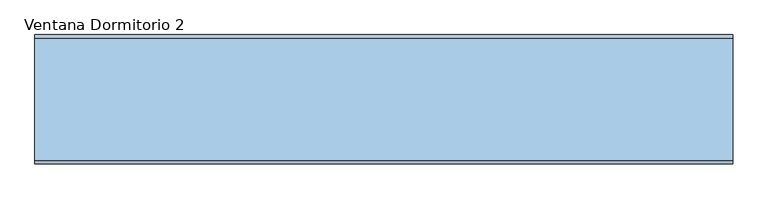
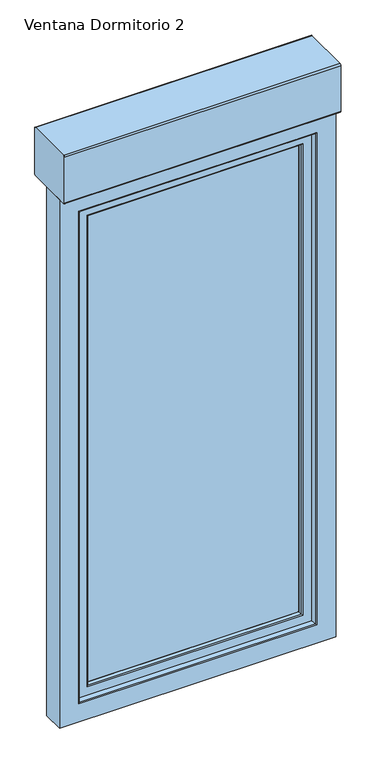
"""IFC4 building model written with IfcOpenShell, lengths in millimetres: window geometry, 2019_ES_Ventana_Replus_re80pvc301_10100_box_1-Hoja_con-Compacto : Ventana Dormitorio 2."""

from ifc_helpers import new_model, si_unit, point, frame, frame_2d, origin, place, context, project, spatial, polyline, circle_curve, ellipse_curve, trimmed, segment, composite_curve, outline, extrude, source, transform, mapped, element, save
from ifc_brep_helpers import plane_surface, cylinder_surface, advanced_brep


def ventana_dormitorio_2_fe78aa6e(model_context):
    return source(origin(), model_context, "Body", "SolidModel", [
        extrude(outline(composite_curve([segment(trimmed(circle_curve(frame_2d((-55.0, 2835.0)), 5.0), [point((-55.0, 2830.0))], [point((-60.0, 2835.0))], False, "CARTESIAN"), True, "CONTINUOUS"), segment(polyline([(-60.0, 2835.0), (-60.0, 3010.0)]), True, "CONTINUOUS"), segment(trimmed(circle_curve(frame_2d((-55.0, 3010.0)), 5.0), [point((-60.0, 3010.0))], [point((-55.0, 3015.0))], False, "CARTESIAN"), True, "CONTINUOUS"), segment(polyline([(-55.0, 3015.0), (120.0, 3015.0)]), True, "CONTINUOUS"), segment(trimmed(circle_curve(frame_2d((120.0, 3010.0)), 5.0), [point((120.0, 3015.0))], [point((125.0, 3010.0))], False, "CARTESIAN"), True, "CONTINUOUS"), segment(polyline([(125.0, 3010.0), (125.0, 2835.0)]), True, "CONTINUOUS"), segment(trimmed(circle_curve(frame_2d((120.0, 2835.0)), 5.0), [point((125.0, 2835.0))], [point((120.0, 2830.0))], False, "CARTESIAN"), True, "CONTINUOUS"), segment(polyline([(120.0, 2830.0), (-55.0, 2830.0)]), True, "CONTINUOUS")], self_intersect=False)), frame((-500.0, 0.0, 0.0), z_axis=(1.0, 0.0, 0.0), x_axis=(0.0, 1.0, 0.0)), (0.0, 0.0, 1.0), 1000.0),
        extrude(outline(polyline([(78.4999991, 1470.0), (118.4999991, 1470.0), (118.4999991, 1360.0), (98.4999991, 1360.0), (98.4999991, 1450.0), (78.4999991, 1450.0), (78.4999991, 1470.0)])), frame((-434.1999993, 0.0, 0.0), z_axis=(1.0, 0.0, 0.0), x_axis=(0.0, 1.0, 0.0)), (0.0, 0.0, 1.0), 12.0),
        extrude(outline(polyline([(-413.9687607, 78.4999991), (-413.9687607, 68.4999991), (-442.4312378, 68.4999991), (-442.4312378, 78.4999991), (-413.9687607, 78.4999991)])), frame((0.0, 0.0, 1435.217127), z_axis=(0.0, 0.0, 1.0), x_axis=(1.0, 0.0, 0.0)), (0.0, 0.0, 1.0), 49.565746),
        extrude(outline(polyline([(909.8, 397.1999993), (2727.2, 397.1999993), (2727.2, -397.1999993), (909.8, -397.1999993), (909.8, 397.1999993)]), holes=[polyline([(2719.2, 389.1999993), (917.8, 389.1999993), (917.8, -389.1999993), (2719.2, -389.1999993), (2719.2, 389.1999993)])]), frame((0.0, 10.9999999, 0.0), z_axis=(0.0, 1.0, 0.0), x_axis=(0.0, 0.0, 1.0)), (0.0, 0.0, 1.0), 16.0),
        extrude(outline(polyline([(909.8131934, 397.1868058), (2727.1868066, 397.1868058), (2727.1868066, -397.1868058), (909.8131934, -397.1868058), (909.8131934, 397.1868058)]), holes=[polyline([(2719.2, 389.1999993), (917.8, 389.1999993), (917.8, -389.1999993), (2719.2, -389.1999993), (2719.2, 389.1999993)])]), frame((0.0, 31.0000001, 0.0), z_axis=(0.0, 1.0, 0.0), x_axis=(0.0, 0.0, 1.0)), (0.0, 0.0, 1.0), 16.0),
        extrude(outline(polyline([(397.1999993, 6.9999997), (-397.1999993, 6.9999997), (-397.1999993, 10.9999999), (397.1999993, 10.9999999), (397.1999993, 6.9999997)])), frame((0.0, 0.0, 903.7946451), z_axis=(0.0, 0.0, 1.0), x_axis=(1.0, 0.0, 0.0)), (0.0, 0.0, 1.0), 1829.4053549),
        extrude(outline(polyline([(397.1999993, 26.9999999), (-397.1999993, 26.9999999), (-397.1999993, 31.0000001), (397.1999993, 31.0000001), (397.1999993, 26.9999999)])), frame((0.0, 0.0, 903.7946451), z_axis=(0.0, 0.0, 1.0), x_axis=(1.0, 0.0, 0.0)), (0.0, 0.0, 1.0), 1829.4053549),
        extrude(outline(polyline([(397.1999993, 47.0000001), (-397.1999993, 47.0000001), (-397.1999993, 51.0000003), (397.1999993, 51.0000003), (397.1999993, 47.0000001)])), frame((0.0, 0.0, 903.7946451), z_axis=(0.0, 0.0, 1.0), x_axis=(1.0, 0.0, 0.0)), (0.0, 0.0, 1.0), 1829.4053549),
        advanced_brep(
        [(387.2913171, -9.2764571, 2717.2913178), (387.2913171, -9.2764571, 922.7086822), (390.1890946, -11.5, 919.8109047), (390.1890946, -11.5, 2720.1890953), (430.1999993, -11.5, 879.8), (430.1999993, -11.5, 2760.2), (-430.1999993, -11.5, 2760.2), (-430.1999993, -11.5, 879.8), (-390.1890946, -11.5, 919.8109047), (-390.1890946, -11.5, 2720.1890953), (-387.2913171, -9.2764571, 922.7086822), (384.1757968, 2.3508228, 2714.1757976), (384.1757968, 2.3508228, 925.8242024), (-384.1757968, 2.3508228, 925.8242024), (384.6739305, 3.0000033, 2714.6739313), (384.6739305, 3.0000033, 925.3260687), (-384.6739305, 3.0000033, 925.3260687), (391.1999993, 3.0000033, 2721.2), (391.1999993, 3.0000033, 918.8), (-391.1999993, 3.0000033, 918.8), (-391.1999993, 3.0000033, 2721.2), (-384.6739305, 3.0000033, 2714.6739313), (391.1999993, 6.9999997, 2721.2), (391.1999993, 6.9999997, 918.8), (-391.1999993, 6.9999997, 918.8), (411.8162192, 6.9999997, 2741.8162199), (411.8162192, 6.9999997, 898.1837801), (-411.8162192, 6.9999997, 898.1837801), (-411.8162192, 6.9999997, 2741.8162199), (-391.1999993, 6.9999997, 2721.2), (409.1999993, 25.6153717, 2739.2), (409.1999993, 25.6153717, 900.8), (-409.1999993, 25.6153717, 900.8), (409.1999993, 56.4999995, 2739.2), (409.1999993, 56.4999995, 900.8), (-409.1999993, 56.4999995, 900.8), (-409.1999993, 56.4999995, 2739.2), (397.1999993, 56.4999995, 2727.2), (397.1999993, 56.4999995, 912.8), (-397.1999993, 56.4999995, 912.8), (-397.1999993, 56.4999995, 2727.2), (397.1999993, 51.0000003, 2727.2), (397.1999993, 51.0000003, 912.8), (-397.1999993, 51.0000003, 912.8), (-397.1999993, 51.0000003, 2727.2), (386.007687, 51.0000003, 2716.0076877), (386.007687, 51.0000003, 923.9923123), (-386.007687, 51.0000003, 923.9923123), (-386.007687, 51.0000003, 2716.0076877), (385.4940999, 51.6693201, 2715.4941006), (385.4940999, 51.6693201, 924.5058994), (-385.4940999, 51.6693201, 924.5058994), (388.8993918, 64.3780426, 2718.8993925), (388.8993918, 64.3780426, 921.1006075), (-388.8993918, 64.3780426, 921.1006075), (392.6234971, 67.3403297, 2722.6234978), (392.6234971, 67.3403297, 917.3765022), (-392.6234971, 67.3403297, 917.3765022), (405.6488427, 67.7951848, 2735.6488434), (405.6488427, 67.7951848, 904.3511566), (-405.6488427, 67.7951848, 904.3511566), (406.1999993, 67.2629391, 2736.2), (406.1999993, 67.2629391, 903.8), (-406.1999993, 67.2629391, 903.8), (407.4370593, 68.4999991, 2737.43706), (407.4370593, 68.4999991, 902.56294), (-407.4370593, 68.4999991, 902.56294), (460.1999993, 68.4999991, 2790.2), (460.1999993, 68.4999991, 849.8), (-460.1999993, 68.4999991, 849.8), (-460.1999993, 68.4999991, 2790.2), (-407.4370593, 68.4999991, 2737.43706), (463.1999993, 65.4999991, 2793.2), (463.1999993, 65.4999991, 846.8), (-463.1999993, 65.4999991, 846.8), (463.1999993, 50.0, 2793.2), (463.1999993, 50.0, 846.8), (-463.1999993, 50.0, 846.8), (-463.1999993, 50.0, 2793.2), (443.1999993, 50.0, 2773.2), (443.1999993, 50.0, 866.8), (-443.1999993, 50.0, 866.8), (-443.1999993, 50.0, 2773.2), (443.1999993, 11.9999991, 2773.2), (443.1999993, 11.9999991, 866.8), (-443.1999993, 11.9999991, 866.8), (-443.1999993, 11.9999991, 2773.2), (430.1999993, 11.9999991, 2760.2), (430.1999993, 11.9999991, 879.8), (-430.1999993, 11.9999991, 879.8), (-430.1999993, 11.9999991, 2760.2), (-387.2913171, -9.2764571, 2717.2913178), (-384.1757968, 2.3508228, 2714.1757976), (-409.1999993, 25.6153717, 2739.2), (-385.4940999, 51.6693201, 2715.4941006), (-388.8993918, 64.3780426, 2718.8993925), (-392.6234971, 67.3403297, 2722.6234978), (-405.6488427, 67.7951848, 2735.6488434), (-406.1999993, 67.2629391, 2736.2), (-463.1999993, 65.4999991, 2793.2)],
        [
            (0, 1),
            (1, 2, ellipse_curve(frame((390.1890946, -8.5, 919.8109047), z_axis=(0.7071067811865475, 0.0, 0.7071067811865475), x_axis=(-0.7071067811865474, 0.0, 0.7071067811865476)), 4.2426407, 3.0)),
            (2, 3),
            (3, 0, ellipse_curve(frame((390.1890946, -8.5, 2720.1890953), z_axis=(0.7071067811865475, 0.0, -0.7071067811865475), x_axis=(0.7071067811865474, 0.0, 0.7071067811865476)), 4.2426407, 3.0)),
            (4, 5),
            (5, 6),
            (6, 7),
            (7, 4),
            (2, 8),
            (8, 9),
            (9, 3),
            (1, 10),
            (10, 8, ellipse_curve(frame((-390.1890946, -8.5, 919.8109047), z_axis=(0.7071067811865475, 0.0, -0.7071067811865475), x_axis=(0.7071067811865476, 0.0, 0.7071067811865474)), 4.2426407, 3.0)),
            (11, 12),
            (12, 1),
            (0, 11),
            (12, 13),
            (13, 10),
            (14, 15),
            (15, 12, ellipse_curve(frame((384.6739305, 2.4842973, 925.3260687), z_axis=(0.7071067811865475, 0.0, 0.7071067811865475), x_axis=(-0.7071067811865474, 0.0, 0.7071067811865476)), 0.7293184, 0.515706)),
            (11, 14, ellipse_curve(frame((384.6739305, 2.4842973, 2714.6739313), z_axis=(0.7071067811865475, 0.0, -0.7071067811865475), x_axis=(0.7071067811865474, 0.0, 0.7071067811865476)), 0.7293184, 0.515706)),
            (15, 16),
            (16, 13, ellipse_curve(frame((-384.6739305, 2.4842973, 925.3260687), z_axis=(0.7071067811865475, 0.0, -0.7071067811865475), x_axis=(0.7071067811865476, 0.0, 0.7071067811865474)), 0.7293184, 0.515706)),
            (17, 18),
            (18, 19),
            (19, 20),
            (20, 17),
            (14, 21),
            (21, 16),
            (22, 23),
            (23, 18),
            (17, 22),
            (23, 24),
            (24, 19),
            (25, 26),
            (26, 27),
            (27, 28),
            (28, 25),
            (22, 29),
            (29, 24),
            (30, 31),
            (31, 26),
            (25, 30),
            (31, 32),
            (32, 27),
            (33, 34),
            (34, 31),
            (30, 33),
            (34, 35),
            (35, 32),
            (33, 36),
            (36, 35),
            (37, 38),
            (38, 39),
            (39, 40),
            (40, 37),
            (41, 42),
            (42, 38),
            (37, 41),
            (42, 43),
            (43, 39),
            (41, 44),
            (44, 43),
            (45, 46),
            (46, 47),
            (47, 48),
            (48, 45),
            (49, 50),
            (50, 46, ellipse_curve(frame((386.007687, 51.5317048, 923.9923123), z_axis=(0.7071067811865475, 0.0, 0.7071067811865475), x_axis=(-0.7071067811865474, 0.0, 0.7071067811865476)), 0.7519437, 0.5317045)),
            (45, 49, ellipse_curve(frame((386.007687, 51.5317048, 2716.0076877), z_axis=(0.7071067811865475, 0.0, -0.7071067811865475), x_axis=(0.7071067811865474, 0.0, 0.7071067811865476)), 0.7519437, 0.5317045)),
            (50, 51),
            (51, 47, ellipse_curve(frame((-386.007687, 51.5317048, 923.9923123), z_axis=(0.7071067811865475, 0.0, -0.7071067811865475), x_axis=(0.7071067811865476, 0.0, 0.7071067811865474)), 0.7519437, 0.5317045)),
            (52, 53),
            (53, 50),
            (49, 52),
            (53, 54),
            (54, 51),
            (55, 56),
            (56, 53, ellipse_curve(frame((392.7630951, 63.3427664, 917.2369042), z_axis=(0.7071067811865475, 0.0, 0.7071067811865475), x_axis=(-0.7071067811865474, 0.0, 0.7071067811865476)), 5.6568542, 4.0)),
            (52, 55, ellipse_curve(frame((392.7630951, 63.3427664, 2722.7630958), z_axis=(0.7071067811865475, 0.0, -0.7071067811865475), x_axis=(0.7071067811865474, 0.0, 0.7071067811865476)), 5.6568542, 4.0)),
            (56, 57),
            (57, 54, ellipse_curve(frame((-392.7630951, 63.3427664, 917.2369042), z_axis=(0.7071067811865475, 0.0, -0.7071067811865475), x_axis=(0.7071067811865476, 0.0, 0.7071067811865474)), 5.6568542, 4.0)),
            (58, 59),
            (59, 56),
            (55, 58),
            (59, 60),
            (60, 57),
            (61, 62),
            (62, 59, ellipse_curve(frame((405.6674291, 67.2629391, 904.3325701), z_axis=(0.7071067811865475, 0.0, 0.7071067811865475), x_axis=(-0.7071067811865474, 0.0, 0.7071067811865476)), 0.7531679, 0.5325701)),
            (58, 61, ellipse_curve(frame((405.6674291, 67.2629391, 2735.6674299), z_axis=(0.7071067811865475, 0.0, -0.7071067811865475), x_axis=(0.7071067811865474, 0.0, 0.7071067811865476)), 0.7531679, 0.5325701)),
            (62, 63),
            (63, 60, ellipse_curve(frame((-405.6674291, 67.2629391, 904.3325701), z_axis=(0.7071067811865475, 0.0, -0.7071067811865475), x_axis=(0.7071067811865476, 0.0, 0.7071067811865474)), 0.7531679, 0.5325701)),
            (64, 65),
            (65, 62, ellipse_curve(frame((407.4370593, 67.2629391, 902.56294), z_axis=(0.7071067811865475, 0.0, 0.7071067811865475), x_axis=(-0.7071067811865474, 0.0, 0.7071067811865476)), 1.7494671, 1.23706)),
            (61, 64, ellipse_curve(frame((407.4370593, 67.2629391, 2737.43706), z_axis=(0.7071067811865475, 0.0, -0.7071067811865475), x_axis=(0.7071067811865474, 0.0, 0.7071067811865476)), 1.7494671, 1.23706)),
            (65, 66),
            (66, 63, ellipse_curve(frame((-407.4370593, 67.2629391, 902.56294), z_axis=(0.7071067811865475, 0.0, -0.7071067811865475), x_axis=(0.7071067811865476, 0.0, 0.7071067811865474)), 1.7494671, 1.23706)),
            (67, 68),
            (68, 69),
            (69, 70),
            (70, 67),
            (64, 71),
            (71, 66),
            (72, 73),
            (73, 68, ellipse_curve(frame((460.1999993, 65.4999991, 849.8), z_axis=(0.7071067811865475, 0.0, 0.7071067811865475), x_axis=(-0.7071067811865474, 0.0, 0.7071067811865476)), 4.2426407, 3.0)),
            (67, 72, ellipse_curve(frame((460.1999993, 65.4999991, 2790.2), z_axis=(0.7071067811865475, 0.0, -0.7071067811865475), x_axis=(0.7071067811865474, 0.0, 0.7071067811865476)), 4.2426407, 3.0)),
            (73, 74),
            (74, 69, ellipse_curve(frame((-460.1999993, 65.4999991, 849.8), z_axis=(0.7071067811865475, 0.0, -0.7071067811865475), x_axis=(0.7071067811865476, 0.0, 0.7071067811865474)), 4.2426407, 3.0)),
            (75, 76),
            (76, 73),
            (72, 75),
            (76, 77),
            (77, 74),
            (75, 78),
            (78, 77),
            (79, 80),
            (80, 81),
            (81, 82),
            (82, 79),
            (79, 83),
            (83, 84),
            (84, 80),
            (84, 85),
            (85, 81),
            (83, 86),
            (86, 85),
            (87, 88),
            (88, 89),
            (89, 90),
            (90, 87),
            (87, 5),
            (4, 88),
            (7, 89),
            (10, 91),
            (91, 9, ellipse_curve(frame((-390.1890946, -8.5, 2720.1890953), z_axis=(-0.7071067811865475, 0.0, -0.7071067811865475), x_axis=(0.7071067811865474, 0.0, -0.7071067811865476)), 4.2426407, 3.0)),
            (13, 92),
            (92, 91),
            (21, 92, ellipse_curve(frame((-384.6739305, 2.4842973, 2714.6739313), z_axis=(-0.7071067811865475, 0.0, -0.7071067811865475), x_axis=(0.7071067811865474, 0.0, -0.7071067811865476)), 0.7293184, 0.515706)),
            (29, 20),
            (32, 93),
            (93, 28),
            (36, 93),
            (44, 40),
            (51, 94),
            (94, 48, ellipse_curve(frame((-386.007687, 51.5317048, 2716.0076877), z_axis=(-0.7071067811865475, 0.0, -0.7071067811865475), x_axis=(0.7071067811865474, 0.0, -0.7071067811865476)), 0.7519437, 0.5317045)),
            (54, 95),
            (95, 94),
            (57, 96),
            (96, 95, ellipse_curve(frame((-392.7630951, 63.3427664, 2722.7630958), z_axis=(-0.7071067811865475, 0.0, -0.7071067811865475), x_axis=(0.7071067811865474, 0.0, -0.7071067811865476)), 5.6568542, 4.0)),
            (60, 97),
            (97, 96),
            (63, 98),
            (98, 97, ellipse_curve(frame((-405.6674291, 67.2629391, 2735.6674299), z_axis=(-0.7071067811865475, 0.0, -0.7071067811865475), x_axis=(0.7071067811865474, 0.0, -0.7071067811865476)), 0.7531679, 0.5325701)),
            (71, 98, ellipse_curve(frame((-407.4370593, 67.2629391, 2737.43706), z_axis=(-0.7071067811865475, 0.0, -0.7071067811865475), x_axis=(0.7071067811865474, 0.0, -0.7071067811865476)), 1.7494671, 1.23706)),
            (74, 99),
            (99, 70, ellipse_curve(frame((-460.1999993, 65.4999991, 2790.2), z_axis=(-0.7071067811865475, 0.0, -0.7071067811865475), x_axis=(0.7071067811865474, 0.0, -0.7071067811865476)), 4.2426407, 3.0)),
            (78, 99),
            (86, 82),
            (6, 90),
            (91, 0),
            (92, 11),
            (93, 30),
            (94, 49),
            (95, 52),
            (96, 55),
            (97, 58),
            (98, 61),
            (99, 72),
        ],
        [
            cylinder_surface(frame((390.1890946, -8.5, 2793.2), z_axis=(0.0, 0.0, 1.0), x_axis=(-1.0, 0.0, 0.0)), 3.0),
            plane_surface(frame((-430.1999993, -11.5, 2760.2), z_axis=(0.0, -1.0, 0.0), x_axis=(1.0, 0.0, 0.0))),
            cylinder_surface(frame((463.1999993, -8.5, 919.8109047), z_axis=(1.0, 0.0, 0.0), x_axis=(0.0, 0.0, 1.0)), 3.0),
            plane_surface(frame((387.2913171, -9.2764571, 2717.2913178), z_axis=(-0.9659258263570549, -0.2588190448487916, 0.0), x_axis=(0.0, 0.0, -1.0))),
            plane_surface(frame((387.2913171, -9.2764571, 922.7086822), z_axis=(0.0, -0.2588190448487885, 0.9659258263570558), x_axis=(-1.0, 0.0, 0.0))),
            cylinder_surface(frame((384.6739305, 2.4842973, 2793.2), z_axis=(0.0, 0.0, 1.0), x_axis=(-1.0, 0.0, 0.0)), 0.515706),
            cylinder_surface(frame((463.1999993, 2.4842973, 925.3260687), z_axis=(1.0, 0.0, 0.0), x_axis=(0.0, 0.0, 1.0)), 0.515706),
            plane_surface(frame((-384.6739305, 3.0000033, 2714.6739313), z_axis=(0.0, 1.0, 0.0), x_axis=(1.0, 0.0, 0.0))),
            plane_surface(frame((391.1999993, 3.0000033, 2721.2), z_axis=(-1.0, 0.0, 0.0), x_axis=(0.0, 0.0, -1.0))),
            plane_surface(frame((391.1999993, 3.0000033, 918.8), z_axis=(0.0, 0.0, 1.0), x_axis=(-1.0, 0.0, 0.0))),
            plane_surface(frame((-391.1999993, 6.9999997, 2721.2), z_axis=(0.0, 1.0, 0.0), x_axis=(1.0, 0.0, 0.0))),
            plane_surface(frame((411.8162192, 6.9999997, 2741.8162199), z_axis=(-0.9902680687415736, -0.13917310096004265, 0.0), x_axis=(0.0, 0.0, -1.0))),
            plane_surface(frame((411.8162192, 6.9999997, 898.1837801), z_axis=(0.0, -0.13917310096003946, 0.990268068741574), x_axis=(-1.0, 0.0, 0.0))),
            plane_surface(frame((409.1999993, 25.6153717, 2739.2), z_axis=(-1.0, 0.0, 0.0), x_axis=(0.0, 0.0, -1.0))),
            plane_surface(frame((409.1999993, 25.6153717, 900.8), z_axis=(0.0, 0.0, 1.0), x_axis=(-1.0, 0.0, 0.0))),
            plane_surface(frame((-409.1999993, 56.4999995, 2739.2), z_axis=(0.0, -1.0, 0.0), x_axis=(1.0, 0.0, 0.0))),
            plane_surface(frame((397.1999993, 56.4999995, 2727.2), z_axis=(1.0, 0.0, 0.0), x_axis=(0.0, 0.0, -1.0))),
            plane_surface(frame((397.1999993, 56.4999995, 912.8), z_axis=(0.0, 0.0, -1.0), x_axis=(-1.0, 0.0, 0.0))),
            plane_surface(frame((-397.1999993, 51.0000003, 2727.2), z_axis=(0.0, -1.0, 0.0), x_axis=(1.0, 0.0, 0.0))),
            cylinder_surface(frame((386.007687, 51.5317048, 2793.2), z_axis=(0.0, 0.0, 1.0), x_axis=(-1.0, 0.0, 0.0)), 0.5317045),
            cylinder_surface(frame((463.1999993, 51.5317048, 923.9923123), z_axis=(1.0, 0.0, 0.0), x_axis=(0.0, 0.0, 1.0)), 0.5317045),
            plane_surface(frame((385.4940999, 51.6693201, 2715.4941006), z_axis=(-0.9659258262890666, 0.2588190451025272, 0.0), x_axis=(0.0, 0.0, -1.0))),
            plane_surface(frame((385.4940999, 51.6693201, 924.5058994), z_axis=(0.0, 0.2588190451025303, 0.9659258262890658), x_axis=(-1.0, 0.0, 0.0))),
            cylinder_surface(frame((392.7630951, 63.3427664, 2793.2), z_axis=(0.0, 0.0, 1.0), x_axis=(-1.0, 0.0, 0.0)), 4.0),
            cylinder_surface(frame((463.1999993, 63.3427664, 917.2369042), z_axis=(1.0, 0.0, 0.0), x_axis=(0.0, 0.0, 1.0)), 4.0),
            plane_surface(frame((392.6234971, 67.3403297, 2722.6234978), z_axis=(-0.034899496702507804, 0.9993908270190955, 0.0), x_axis=(0.0, 0.0, -1.0))),
            plane_surface(frame((392.6234971, 67.3403297, 917.3765022), z_axis=(0.0, 0.9993908270190957, 0.03489949670250457), x_axis=(-1.0, 0.0, 0.0))),
            cylinder_surface(frame((405.6674291, 67.2629391, 2793.2), z_axis=(0.0, 0.0, 1.0), x_axis=(-1.0, 0.0, 0.0)), 0.5325701),
            cylinder_surface(frame((463.1999993, 67.2629391, 904.3325701), z_axis=(1.0, 0.0, 0.0), x_axis=(0.0, 0.0, 1.0)), 0.5325701),
            cylinder_surface(frame((407.4370593, 67.2629391, 2793.2), z_axis=(0.0, 0.0, 1.0), x_axis=(-1.0, 0.0, 0.0)), 1.23706),
            cylinder_surface(frame((463.1999993, 67.2629391, 902.56294), z_axis=(1.0, 0.0, 0.0), x_axis=(0.0, 0.0, 1.0)), 1.23706),
            plane_surface(frame((-407.4370593, 68.4999991, 2737.43706), z_axis=(0.0, 1.0, 0.0), x_axis=(1.0, 0.0, 0.0))),
            cylinder_surface(frame((460.1999993, 65.4999991, 2793.2), z_axis=(0.0, 0.0, 1.0), x_axis=(-1.0, 0.0, 0.0)), 3.0),
            cylinder_surface(frame((463.1999993, 65.4999991, 849.8), z_axis=(1.0, 0.0, 0.0), x_axis=(0.0, 0.0, 1.0)), 3.0),
            plane_surface(frame((463.1999993, 65.4999991, 2793.2), z_axis=(1.0, 0.0, 0.0), x_axis=(0.0, 0.0, -1.0))),
            plane_surface(frame((463.1999993, 65.4999991, 846.8), z_axis=(0.0, 0.0, -1.0), x_axis=(-1.0, 0.0, 0.0))),
            plane_surface(frame((-459.2000019, 50.0, 2789.2000027), z_axis=(0.0, -1.0, 0.0), x_axis=(1.0, 0.0, 0.0))),
            plane_surface(frame((443.1999993, 45.0999991, 2773.2), z_axis=(1.0, 0.0, 0.0), x_axis=(0.0, 0.0, -1.0))),
            plane_surface(frame((443.1999993, 45.0999991, 866.8), z_axis=(0.0, 0.0, -1.0), x_axis=(-1.0, 0.0, 0.0))),
            plane_surface(frame((-435.7000002, 11.9999991, 2765.7000009), z_axis=(0.0, -1.0, 0.0), x_axis=(1.0, 0.0, 0.0))),
            plane_surface(frame((430.1999993, 1.4999991, 2760.2), z_axis=(1.0, 0.0, 0.0), x_axis=(0.0, 0.0, -1.0))),
            plane_surface(frame((430.1999993, 1.4999991, 879.8), z_axis=(0.0, 0.0, -1.0), x_axis=(-1.0, 0.0, 0.0))),
            cylinder_surface(frame((-390.1890946, -8.5, 846.8), z_axis=(0.0, 0.0, -1.0), x_axis=(1.0, 0.0, 0.0)), 3.0),
            plane_surface(frame((-387.2913171, -9.2764571, 922.7086822), z_axis=(0.9659258263570565, -0.2588190448487853, 0.0), x_axis=(0.0, 0.0, 1.0))),
            cylinder_surface(frame((-384.6739305, 2.4842973, 846.8), z_axis=(0.0, 0.0, -1.0), x_axis=(1.0, 0.0, 0.0)), 0.515706),
            plane_surface(frame((-391.1999993, 3.0000033, 918.8), z_axis=(1.0, 0.0, 0.0), x_axis=(0.0, 0.0, 1.0))),
            plane_surface(frame((-411.8162192, 6.9999997, 898.1837801), z_axis=(0.9902680687415745, -0.13917310096003627, 0.0), x_axis=(0.0, 0.0, 1.0))),
            plane_surface(frame((-409.1999993, 25.6153717, 900.8), z_axis=(1.0, 0.0, 0.0), x_axis=(0.0, 0.0, 1.0))),
            plane_surface(frame((-397.1999993, 56.4999995, 912.8), z_axis=(-1.0, 0.0, 0.0), x_axis=(0.0, 0.0, 1.0))),
            cylinder_surface(frame((-386.007687, 51.5317048, 846.8), z_axis=(0.0, 0.0, -1.0), x_axis=(1.0, 0.0, 0.0)), 0.5317045),
            plane_surface(frame((-385.4940999, 51.6693201, 924.5058994), z_axis=(0.9659258262890649, 0.2588190451025334, 0.0), x_axis=(0.0, 0.0, 1.0))),
            cylinder_surface(frame((-392.7630951, 63.3427664, 846.8), z_axis=(0.0, 0.0, -1.0), x_axis=(1.0, 0.0, 0.0)), 4.0),
            plane_surface(frame((-392.6234971, 67.3403297, 917.3765022), z_axis=(0.03489949670250134, 0.9993908270190958, 0.0), x_axis=(0.0, 0.0, 1.0))),
            cylinder_surface(frame((-405.6674291, 67.2629391, 846.8), z_axis=(0.0, 0.0, -1.0), x_axis=(1.0, 0.0, 0.0)), 0.5325701),
            cylinder_surface(frame((-407.4370593, 67.2629391, 846.8), z_axis=(0.0, 0.0, -1.0), x_axis=(1.0, 0.0, 0.0)), 1.23706),
            cylinder_surface(frame((-460.1999993, 65.4999991, 846.8), z_axis=(0.0, 0.0, -1.0), x_axis=(1.0, 0.0, 0.0)), 3.0),
            plane_surface(frame((-463.1999993, 65.4999991, 846.8), z_axis=(-1.0, 0.0, 0.0), x_axis=(0.0, 0.0, 1.0))),
            plane_surface(frame((-443.1999993, 45.0999991, 866.8), z_axis=(-1.0, 0.0, 0.0), x_axis=(0.0, 0.0, 1.0))),
            plane_surface(frame((-430.1999993, 1.4999991, 879.8), z_axis=(-1.0, 0.0, 0.0), x_axis=(0.0, 0.0, 1.0))),
            cylinder_surface(frame((-463.1999993, -8.5, 2720.1890953), z_axis=(-1.0, 0.0, 0.0), x_axis=(0.0, 0.0, -1.0)), 3.0),
            plane_surface(frame((-387.2913171, -9.2764571, 2717.2913178), z_axis=(0.0, -0.2588190448487885, -0.9659258263570557), x_axis=(1.0, 0.0, 0.0))),
            cylinder_surface(frame((-463.1999993, 2.4842973, 2714.6739313), z_axis=(-1.0, 0.0, 0.0), x_axis=(0.0, 0.0, -1.0)), 0.515706),
            plane_surface(frame((-391.1999993, 3.0000033, 2721.2), z_axis=(0.0, 0.0, -1.0), x_axis=(1.0, 0.0, 0.0))),
            plane_surface(frame((-411.8162192, 6.9999997, 2741.8162199), z_axis=(0.0, -0.13917310096003946, -0.990268068741574), x_axis=(1.0, 0.0, 0.0))),
            plane_surface(frame((-409.1999993, 25.6153717, 2739.2), z_axis=(0.0, 0.0, -1.0), x_axis=(1.0, 0.0, 0.0))),
            plane_surface(frame((-397.1999993, 56.4999995, 2727.2), z_axis=(0.0, 0.0, 1.0), x_axis=(1.0, 0.0, 0.0))),
            cylinder_surface(frame((-463.1999993, 51.5317048, 2716.0076877), z_axis=(-1.0, 0.0, 0.0), x_axis=(0.0, 0.0, -1.0)), 0.5317045),
            plane_surface(frame((-385.4940999, 51.6693201, 2715.4941006), z_axis=(0.0, 0.2588190451025303, -0.9659258262890658), x_axis=(1.0, 0.0, 0.0))),
            cylinder_surface(frame((-463.1999993, 63.3427664, 2722.7630958), z_axis=(-1.0, 0.0, 0.0), x_axis=(0.0, 0.0, -1.0)), 4.0),
            plane_surface(frame((-392.6234971, 67.3403297, 2722.6234978), z_axis=(0.0, 0.9993908270190957, -0.03489949670250457), x_axis=(1.0, 0.0, 0.0))),
            cylinder_surface(frame((-463.1999993, 67.2629391, 2735.6674299), z_axis=(-1.0, 0.0, 0.0), x_axis=(0.0, 0.0, -1.0)), 0.5325701),
            cylinder_surface(frame((-463.1999993, 67.2629391, 2737.43706), z_axis=(-1.0, 0.0, 0.0), x_axis=(0.0, 0.0, -1.0)), 1.23706),
            cylinder_surface(frame((-463.1999993, 65.4999991, 2790.2), z_axis=(-1.0, 0.0, 0.0), x_axis=(0.0, 0.0, -1.0)), 3.0),
            plane_surface(frame((-463.1999993, 65.4999991, 2793.2), z_axis=(0.0, 0.0, 1.0), x_axis=(1.0, 0.0, 0.0))),
            plane_surface(frame((-443.1999993, 45.0999991, 2773.2), z_axis=(0.0, 0.0, 1.0), x_axis=(1.0, 0.0, 0.0))),
            plane_surface(frame((-430.1999993, 1.4999991, 2760.2), z_axis=(0.0, 0.0, 1.0), x_axis=(1.0, 0.0, 0.0))),
        ],
        [
            (0, [[1, 2, 3, 4]]),
            (1, [[5, 6, 7, 8], [-3, 9, 10, 11]]),
            (2, [[12, 13, -9, -2]]),
            (3, [[14, 15, -1, 16]]),
            (4, [[17, 18, -12, -15]]),
            (5, [[19, 20, -14, 21]]),
            (6, [[22, 23, -17, -20]]),
            (7, [[24, 25, 26, 27], [-19, 28, 29, -22]]),
            (8, [[30, 31, -24, 32]]),
            (9, [[33, 34, -25, -31]]),
            (10, [[35, 36, 37, 38], [-30, 39, 40, -33]]),
            (11, [[41, 42, -35, 43]]),
            (12, [[44, 45, -36, -42]]),
            (13, [[46, 47, -41, 48]]),
            (14, [[49, 50, -44, -47]]),
            (15, [[-46, 51, 52, -49], [53, 54, 55, 56]]),
            (16, [[57, 58, -53, 59]]),
            (17, [[60, 61, -54, -58]]),
            (18, [[-57, 62, 63, -60], [64, 65, 66, 67]]),
            (19, [[68, 69, -64, 70]]),
            (20, [[71, 72, -65, -69]]),
            (21, [[73, 74, -68, 75]]),
            (22, [[76, 77, -71, -74]]),
            (23, [[78, 79, -73, 80]]),
            (24, [[81, 82, -76, -79]]),
            (25, [[83, 84, -78, 85]]),
            (26, [[86, 87, -81, -84]]),
            (27, [[88, 89, -83, 90]]),
            (28, [[91, 92, -86, -89]]),
            (29, [[93, 94, -88, 95]]),
            (30, [[96, 97, -91, -94]]),
            (31, [[98, 99, 100, 101], [-93, 102, 103, -96]]),
            (32, [[104, 105, -98, 106]]),
            (33, [[107, 108, -99, -105]]),
            (34, [[109, 110, -104, 111]]),
            (35, [[112, 113, -107, -110]]),
            (36, [[-109, 114, 115, -112], [116, 117, 118, 119]]),
            (37, [[120, 121, 122, -116]]),
            (38, [[123, 124, -117, -122]]),
            (39, [[-121, 125, 126, -123], [127, 128, 129, 130]]),
            (40, [[131, -5, 132, -127]]),
            (41, [[-8, 133, -128, -132]]),
            (42, [[134, 135, -10, -13]]),
            (43, [[136, 137, -134, -18]]),
            (44, [[-29, 138, -136, -23]]),
            (45, [[-40, 139, -26, -34]]),
            (46, [[140, 141, -37, -45]]),
            (47, [[-52, 142, -140, -50]]),
            (48, [[-63, 143, -55, -61]]),
            (49, [[144, 145, -66, -72]]),
            (50, [[146, 147, -144, -77]]),
            (51, [[148, 149, -146, -82]]),
            (52, [[150, 151, -148, -87]]),
            (53, [[152, 153, -150, -92]]),
            (54, [[-103, 154, -152, -97]]),
            (55, [[155, 156, -100, -108]]),
            (56, [[-115, 157, -155, -113]]),
            (57, [[-126, 158, -118, -124]]),
            (58, [[-7, 159, -129, -133]]),
            (59, [[160, -4, -11, -135]]),
            (60, [[161, -16, -160, -137]]),
            (61, [[-28, -21, -161, -138]]),
            (62, [[-39, -32, -27, -139]]),
            (63, [[162, -43, -38, -141]]),
            (64, [[-51, -48, -162, -142]]),
            (65, [[-62, -59, -56, -143]]),
            (66, [[163, -70, -67, -145]]),
            (67, [[164, -75, -163, -147]]),
            (68, [[165, -80, -164, -149]]),
            (69, [[166, -85, -165, -151]]),
            (70, [[167, -90, -166, -153]]),
            (71, [[-102, -95, -167, -154]]),
            (72, [[168, -106, -101, -156]]),
            (73, [[-114, -111, -168, -157]]),
            (74, [[-125, -120, -119, -158]]),
            (75, [[-6, -131, -130, -159]]),
        ],
    ),
        advanced_brep(
        [(423.2673545, -12.758819, 2753.2673545), (423.2673545, -12.758819, 886.7326455), (427.2913185, -27.7764571, 882.7086815), (427.2913185, -27.7764571, 2757.2913185), (430.189096, -30.0, 879.810904), (430.189096, -30.0, 2760.189096), (-423.2673545, -12.758819, 886.7326455), (-427.2913185, -27.7764571, 882.7086815), (424.2332803, -11.5, 2754.2332803), (424.2332803, -11.5, 885.7667197), (500.0, -30.0, 2830.0), (500.0, -30.0, 810.0), (500.0, 50.0, 810.0), (500.0, 50.0, 2830.0), (-500.0, 50.0, 810.0), (-500.0, 50.0, 2830.0), (456.1999993, 50.0, 853.8000007), (456.1999993, 50.0, 2786.1999993), (-456.1999993, 50.0, 2786.1999993), (-456.1999993, 50.0, 853.8000007), (-500.0, -30.0, 810.0), (-500.0, -30.0, 2830.0), (-430.189096, -30.0, 879.810904), (-430.189096, -30.0, 2760.189096), (436.1891471, 8.0, 2766.1891471), (436.1891471, 8.0, 873.8108529), (436.1891471, -11.5, 873.8108529), (436.1891471, -11.5, 2766.1891471), (-436.1891471, -11.5, 873.8108529), (-436.1891471, -11.5, 2766.1891471), (-424.2332803, -11.5, 2754.2332803), (-424.2332803, -11.5, 885.7667197), (-436.1891471, 8.0, 873.8108529), (455.1999993, 8.0, 2785.1999993), (455.1999993, 8.0, 854.8000007), (-455.1999993, 8.0, 854.8000007), (-455.1999993, 8.0, 2785.1999993), (-436.1891471, 8.0, 2766.1891471), (455.1999993, 49.0, 854.8000007), (455.1999993, 49.0, 2785.1999993), (-455.1999993, 49.0, 854.8000007), (-423.2673545, -12.758819, 2753.2673545), (-427.2913185, -27.7764571, 2757.2913185), (-455.1999993, 49.0, 2785.1999993)],
        [
            (0, 1),
            (1, 2),
            (2, 3),
            (3, 0),
            (2, 4, ellipse_curve(frame((430.189096, -27.0, 879.810904), z_axis=(0.7071067811865475, 0.0, 0.7071067811865475), x_axis=(-0.7071067811865474, 0.0, 0.7071067811865476)), 4.2426407, 3.0)),
            (4, 5),
            (5, 3, ellipse_curve(frame((430.189096, -27.0, 2760.189096), z_axis=(0.7071067811865475, 0.0, -0.7071067811865475), x_axis=(0.7071067811865474, 0.0, 0.7071067811865476)), 4.2426407, 3.0)),
            (1, 6),
            (6, 7),
            (7, 2),
            (8, 9),
            (9, 1, ellipse_curve(frame((424.2332803, -12.5, 885.7667197), z_axis=(0.7071067811865475, 0.0, 0.7071067811865475), x_axis=(-0.7071067811865474, 0.0, 0.7071067811865476)), 1.4142136, 1.0)),
            (0, 8, ellipse_curve(frame((424.2332803, -12.5, 2754.2332803), z_axis=(0.7071067811865475, 0.0, -0.7071067811865475), x_axis=(0.7071067811865474, 0.0, 0.7071067811865476)), 1.4142136, 1.0)),
            (10, 11),
            (11, 12),
            (12, 13),
            (13, 10),
            (12, 14),
            (14, 15),
            (15, 13),
            (16, 17),
            (17, 18),
            (18, 19),
            (19, 16),
            (11, 20),
            (20, 14),
            (10, 21),
            (21, 20),
            (4, 22),
            (22, 23),
            (23, 5),
            (24, 25),
            (25, 26),
            (26, 27),
            (27, 24),
            (26, 28),
            (28, 29),
            (29, 27),
            (8, 30),
            (30, 31),
            (31, 9),
            (25, 32),
            (32, 28),
            (33, 34),
            (34, 35),
            (35, 36),
            (36, 33),
            (24, 37),
            (37, 32),
            (16, 38, ellipse_curve(frame((456.1999993, 49.0, 853.8000007), z_axis=(0.7071067811865475, 0.0, 0.7071067811865475), x_axis=(-0.7071067811865474, 0.0, 0.7071067811865476)), 1.4142136, 1.0)),
            (38, 39),
            (39, 17, ellipse_curve(frame((456.1999993, 49.0, 2786.1999993), z_axis=(0.7071067811865475, 0.0, -0.7071067811865475), x_axis=(0.7071067811865474, 0.0, 0.7071067811865476)), 1.4142136, 1.0)),
            (38, 34),
            (33, 39),
            (19, 40, ellipse_curve(frame((-456.1999993, 49.0, 853.8000007), z_axis=(0.7071067811865475, 0.0, -0.7071067811865475), x_axis=(0.7071067811865476, 0.0, 0.7071067811865474)), 1.4142136, 1.0)),
            (40, 38),
            (31, 6, ellipse_curve(frame((-424.2332803, -12.5, 885.7667197), z_axis=(0.7071067811865475, 0.0, -0.7071067811865475), x_axis=(0.7071067811865476, 0.0, 0.7071067811865474)), 1.4142136, 1.0)),
            (7, 22, ellipse_curve(frame((-430.189096, -27.0, 879.810904), z_axis=(0.7071067811865475, 0.0, -0.7071067811865475), x_axis=(0.7071067811865476, 0.0, 0.7071067811865474)), 4.2426407, 3.0)),
            (6, 41),
            (41, 42),
            (42, 7),
            (21, 15),
            (37, 29),
            (40, 35),
            (18, 43, ellipse_curve(frame((-456.1999993, 49.0, 2786.1999993), z_axis=(-0.7071067811865475, 0.0, -0.7071067811865475), x_axis=(0.7071067811865474, 0.0, -0.7071067811865476)), 1.4142136, 1.0)),
            (43, 40),
            (30, 41, ellipse_curve(frame((-424.2332803, -12.5, 2754.2332803), z_axis=(-0.7071067811865475, 0.0, -0.7071067811865475), x_axis=(0.7071067811865474, 0.0, -0.7071067811865476)), 1.4142136, 1.0)),
            (42, 23, ellipse_curve(frame((-430.189096, -27.0, 2760.189096), z_axis=(-0.7071067811865475, 0.0, -0.7071067811865475), x_axis=(0.7071067811865474, 0.0, -0.7071067811865476)), 4.2426407, 3.0)),
            (43, 36),
            (41, 0),
            (3, 42),
            (39, 43),
        ],
        [
            plane_surface(frame((427.2913185, -27.7764571, 2757.2913185), z_axis=(-0.9659258262890693, -0.2588190451025169, 0.0), x_axis=(0.0, 0.0, -1.0))),
            cylinder_surface(frame((430.189096, -27.0, 2830.0), z_axis=(0.0, 0.0, 1.0), x_axis=(-1.0, 0.0, 0.0)), 3.0),
            plane_surface(frame((427.2913185, -27.7764571, 882.7086815), z_axis=(0.0, -0.2588190451025138, 0.9659258262890702), x_axis=(-1.0, 0.0, 0.0))),
            cylinder_surface(frame((424.2332803, -12.5, 2830.0), z_axis=(0.0, 0.0, 1.0), x_axis=(-1.0, 0.0, 0.0)), 1.0),
            plane_surface(frame((500.0, 50.0, 2830.0), z_axis=(1.0, 0.0, 0.0), x_axis=(0.0, 0.0, -1.0))),
            plane_surface(frame((-456.1999993, 50.0, 2786.1999993), z_axis=(0.0, 1.0, 0.0), x_axis=(1.0, 0.0, 0.0))),
            plane_surface(frame((500.0, 50.0, 810.0), z_axis=(0.0, 0.0, -1.0), x_axis=(-1.0, 0.0, 0.0))),
            plane_surface(frame((-500.0, -30.0, 2830.0), z_axis=(0.0, -1.0, 0.0), x_axis=(1.0, 0.0, 0.0))),
            plane_surface(frame((436.1891471, -11.5, 2766.1891471), z_axis=(-1.0, 0.0, 0.0), x_axis=(0.0, 0.0, -1.0))),
            plane_surface(frame((-424.2332803, -11.5, 2754.2332803), z_axis=(0.0, 1.0, 0.0), x_axis=(1.0, 0.0, 0.0))),
            plane_surface(frame((436.1891471, -11.5, 873.8108529), z_axis=(0.0, 0.0, 1.0), x_axis=(-1.0, 0.0, 0.0))),
            plane_surface(frame((-436.1891471, 8.0, 2766.1891471), z_axis=(0.0, 1.0, 0.0), x_axis=(1.0, 0.0, 0.0))),
            cylinder_surface(frame((456.1999993, 49.0, 2830.0), z_axis=(0.0, 0.0, 1.0), x_axis=(-1.0, 0.0, 0.0)), 1.0),
            plane_surface(frame((455.1999993, 8.0, 2785.1999993), z_axis=(-1.0, 0.0, 0.0), x_axis=(0.0, 0.0, -1.0))),
            cylinder_surface(frame((500.0, 49.0, 853.8000007), z_axis=(1.0, 0.0, 0.0), x_axis=(0.0, 0.0, 1.0)), 1.0),
            cylinder_surface(frame((500.0, -12.5, 885.7667197), z_axis=(1.0, 0.0, 0.0), x_axis=(0.0, 0.0, 1.0)), 1.0),
            cylinder_surface(frame((500.0, -27.0, 879.810904), z_axis=(1.0, 0.0, 0.0), x_axis=(0.0, 0.0, 1.0)), 3.0),
            plane_surface(frame((-427.2913185, -27.7764571, 882.7086815), z_axis=(0.9659258262890711, -0.2588190451025107, 0.0), x_axis=(0.0, 0.0, 1.0))),
            plane_surface(frame((-500.0, 50.0, 810.0), z_axis=(-1.0, 0.0, 0.0), x_axis=(0.0, 0.0, 1.0))),
            plane_surface(frame((-436.1891471, -11.5, 873.8108529), z_axis=(1.0, 0.0, 0.0), x_axis=(0.0, 0.0, 1.0))),
            plane_surface(frame((455.1999993, 8.0, 854.8000007), z_axis=(0.0, 0.0, 1.0), x_axis=(-1.0, 0.0, 0.0))),
            cylinder_surface(frame((-456.1999993, 49.0, 810.0), z_axis=(0.0, 0.0, -1.0), x_axis=(1.0, 0.0, 0.0)), 1.0),
            cylinder_surface(frame((-424.2332803, -12.5, 810.0), z_axis=(0.0, 0.0, -1.0), x_axis=(1.0, 0.0, 0.0)), 1.0),
            cylinder_surface(frame((-430.189096, -27.0, 810.0), z_axis=(0.0, 0.0, -1.0), x_axis=(1.0, 0.0, 0.0)), 3.0),
            plane_surface(frame((-455.1999993, 8.0, 854.8000007), z_axis=(1.0, 0.0, 0.0), x_axis=(0.0, 0.0, 1.0))),
            plane_surface(frame((-427.2913185, -27.7764571, 2757.2913185), z_axis=(0.0, -0.2588190451025138, -0.9659258262890702), x_axis=(1.0, 0.0, 0.0))),
            plane_surface(frame((-500.0, 50.0, 2830.0), z_axis=(0.0, 0.0, 1.0), x_axis=(1.0, 0.0, 0.0))),
            plane_surface(frame((-436.1891471, -11.5, 2766.1891471), z_axis=(0.0, 0.0, -1.0), x_axis=(1.0, 0.0, 0.0))),
            cylinder_surface(frame((-500.0, 49.0, 2786.1999993), z_axis=(-1.0, 0.0, 0.0), x_axis=(0.0, 0.0, -1.0)), 1.0),
            cylinder_surface(frame((-500.0, -12.5, 2754.2332803), z_axis=(-1.0, 0.0, 0.0), x_axis=(0.0, 0.0, -1.0)), 1.0),
            cylinder_surface(frame((-500.0, -27.0, 2760.189096), z_axis=(-1.0, 0.0, 0.0), x_axis=(0.0, 0.0, -1.0)), 3.0),
            plane_surface(frame((-455.1999993, 8.0, 2785.1999993), z_axis=(0.0, 0.0, -1.0), x_axis=(1.0, 0.0, 0.0))),
        ],
        [
            (0, [[1, 2, 3, 4]]),
            (1, [[-3, 5, 6, 7]]),
            (2, [[8, 9, 10, -2]]),
            (3, [[11, 12, -1, 13]]),
            (4, [[14, 15, 16, 17]]),
            (5, [[-16, 18, 19, 20], [21, 22, 23, 24]]),
            (6, [[25, 26, -18, -15]]),
            (7, [[-14, 27, 28, -25], [-6, 29, 30, 31]]),
            (8, [[32, 33, 34, 35]]),
            (9, [[-34, 36, 37, 38], [-11, 39, 40, 41]]),
            (10, [[42, 43, -36, -33]]),
            (11, [[44, 45, 46, 47], [-32, 48, 49, -42]]),
            (12, [[-21, 50, 51, 52]]),
            (13, [[-51, 53, -44, 54]]),
            (14, [[-24, 55, 56, -50]]),
            (15, [[-41, 57, -8, -12]]),
            (16, [[-10, 58, -29, -5]]),
            (17, [[59, 60, 61, -9]]),
            (18, [[-28, 62, -19, -26]]),
            (19, [[-49, 63, -37, -43]]),
            (20, [[-56, 64, -45, -53]]),
            (21, [[-23, 65, 66, -55]]),
            (22, [[-40, 67, -59, -57]]),
            (23, [[-61, 68, -30, -58]]),
            (24, [[-66, 69, -46, -64]]),
            (25, [[70, -4, 71, -60]]),
            (26, [[-27, -17, -20, -62]]),
            (27, [[-48, -35, -38, -63]]),
            (28, [[-22, -52, 72, -65]]),
            (29, [[-39, -13, -70, -67]]),
            (30, [[-71, -7, -31, -68]]),
            (31, [[-72, -54, -47, -69]]),
        ],
    ),
    ])


if __name__ == "__main__":
    model = new_model("IFC4")
    model_context = context("Model", 3, world=origin())
    ifc_project = project(units=[si_unit("LENGTHUNIT", "METRE", prefix="MILLI")], contexts=[model_context])
    site = spatial("IfcSite", under=ifc_project)
    building = spatial("IfcBuilding", under=site)
    placement = place(None, origin())
    ventana_dormitorio_2_shape = ventana_dormitorio_2_fe78aa6e(model_context)
    element("IfcWindow", 1, ObjectType="2019_ES_Ventana_Replus_re80pvc301_10100_box_1-Hoja_con-Compacto : Ventana Dormitorio 2", at=placement, inside=building, context=model_context, shape_type="MappedRepresentation", body=[
        mapped(ventana_dormitorio_2_shape, transform((0.0, 0.0, 0.0), x_axis=(1.0, 0.0, 0.0), y_axis=(0.0, 1.0, 0.0), z_axis=(0.0, 0.0, 1.0))),
    ])
    save(model, "model.ifc")

# Revit data of these elements
# Type "2019_ES_Ventana_Replus_re80pvc301_10100_box_1-Hoja_con-Compacto : Ventana Dormitorio 2"
#   Type Mark = "45"
#   URL = "https://replus.es/"
#   Product data url = "https://bimetica.com/es/objetos-bim-replus-ventana-practicable-oscilobatiente-una-hoja-con-compacto-9540"
#   Product Guid = ""
#   Model = "10100 BOX"
#   Material secondary = "Glass"
#   Material main = "PVC"
#   Manufacturer = "Replus"
#   Keynote = "08500"
#   EAN code = ""
#   Description = "Perfiles de PVC con triple junta (por junta rígida en el marco). Protegiendo de este modo todos los puntos de cierre y proporcionando una junta perimetral completa, con un grosor en el perfil de 3 mm. Vidrio de alta calidad con diferentes posibilidades"
#   Assembly Code = "B2020100"
#   Analytic Construction = "<None>"
#   Ι_Wll Thcknss [instance default] = 20.0 cm
#   Ι_Wdth Cntrl = 100.0 cm
#   Ι_Nst Cntrl [instance default] = 0.0 cm
#   Ι_Hndl Hght Cntrl = 65.0 cm
#   Ι_Hght Cntrl = 202.0 cm
#   Rough Width = 102.0 cm
#   Rough Height = 204.0 cm
#   Retranqueo [instance default] = 0.0 cm
#   I_Lf_Cntrl = 92.64 cm
#   Hueco = 1.0 cm
#   Height = 202.0 cm
#   Default Sill Height = 80.0 cm
#   Width = 100.0 cm
#   Altura de Manilla = 65.0 cm
#   Visibilidad Líneas Apertura - Planta = yes
#   Visibilidad Líneas Apertura - Alzado = yes
#   Exceso Dimensiones = no
#   Edition number = 1
#   Advertencia Dimensión = yes
#   Product Material = PVC - Replus - 9152 - White
#   Wall Closure = (empty or 0)
# Element 1 (IfcWindow, "2019_ES_Ventana_Replus_re80pvc301_10100_box_1-Hoja_con-Compacto : Ventana Dormitorio 2")
#   Ι_Wll Thcknss = 10.0 cm
#   Materials on its faces: "PVC - Replus - 9152 - White", "Rubber - Replus - Black", "Glass - Replus"
# Materials
#   "PVC - Replus - 9152 - White": class "Miscellaneous", colour RGB 174 174 166, transparency 0, Manufacturer = "Replus", Comments = "Rendering appearance not upgraded ", URL = "https://replus.es/", Cost = 0
#   "Rubber - Replus - Black": class "Plastic", colour RGB 63 63 63, transparency 0, Description = "Natural rubber, black", Cost = 0
#   "Glass - Replus": class "Glass", colour RGB 218 227 224, transparency 0.85, Cost = 0
